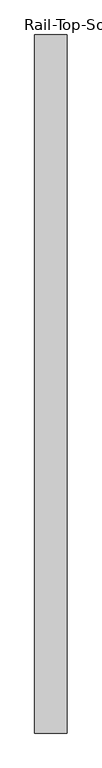
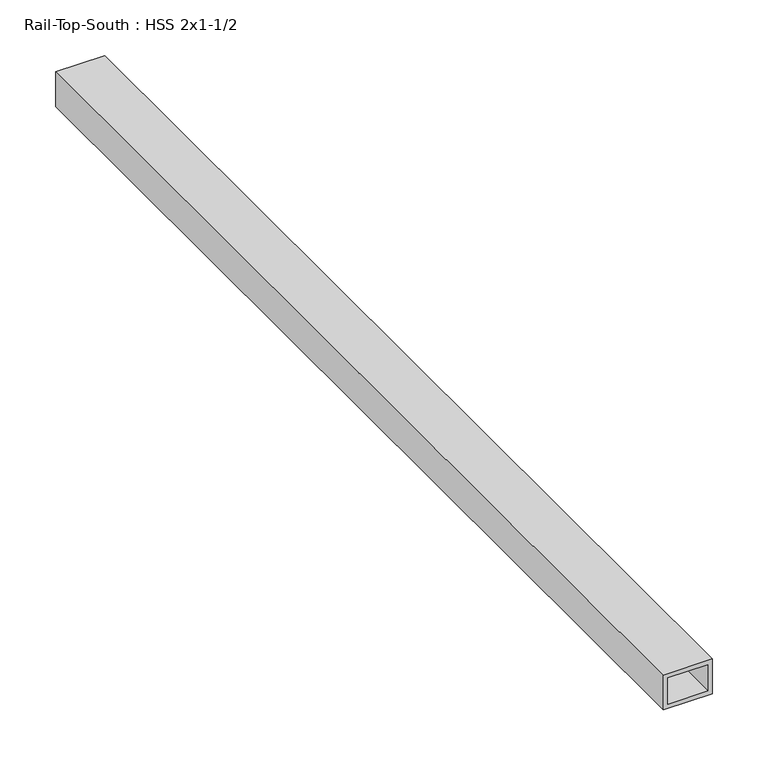
"""IFC4 building model written with IfcOpenShell, lengths in millimetres: proxy geometry, Rail-Top-South : HSS 2x1-1/2."""

from ifc_helpers import new_model, si_unit, frame, origin, place, context, project, spatial, polyline, outline, extrude, source, transform, mapped, element, save


def rail_top_south_hss_2x1_1_2_0885d97b(model_context):
    return source(origin(), model_context, "Body", "SweptSolid", [
        extrude(outline(polyline([(2400.3, 587416.6934739), (2438.4, 587416.6934739), (2438.4, 587365.8934739), (2400.3, 587365.8934739), (2400.3, 587416.6934739)]), holes=[polyline([(2433.6375, 587411.9309739), (2405.0625, 587411.9309739), (2405.0625, 587370.6559739), (2433.6375, 587370.6559739), (2433.6375, 587411.9309739)])]), frame((0.0, -533976.0163841, 0.0), z_axis=(0.0, 1.0, 0.0), x_axis=(0.0, 0.0, 1.0)), (0.0, 0.0, 1.0), 1092.2),
    ])


if __name__ == "__main__":
    model = new_model("IFC4")
    model_context = context("Model", 3, world=origin())
    ifc_project = project(units=[si_unit("LENGTHUNIT", "METRE", prefix="MILLI")], contexts=[model_context])
    site = spatial("IfcSite", under=ifc_project)
    building = spatial("IfcBuilding", under=site)
    placement = place(None, origin())
    rail_top_south_hss_2x1_1_2_shape = rail_top_south_hss_2x1_1_2_0885d97b(model_context)
    element("IfcBuildingElementProxy", 1, Name="Rail-Top-South : HSS 2x1-1/2", ObjectType="Rail-Top-South : HSS 2x1-1/2", at=placement, inside=building, context=model_context, shape_type="MappedRepresentation", body=[
        mapped(rail_top_south_hss_2x1_1_2_shape, transform((0.0, 0.0, 0.0), x_axis=(1.0, 0.0, 0.0), y_axis=(0.0, 1.0, 0.0), z_axis=(0.0, 0.0, 1.0))),
    ])
    save(model, "model.ifc")

# Revit data of these elements
# Element 1 (IfcBuildingElementProxy, "Rail-Top-South : HSS 2x1-1/2")
#   Materials on its faces: "1-1/2\"X2\" GALV. STL HSS TUBING"
# Materials
#   "1-1/2\"X2\" GALV. STL HSS TUBING": class "Generic", colour RGB 211 211 207, transparency 0, Cost = 0
